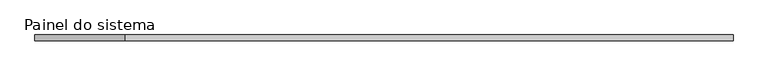
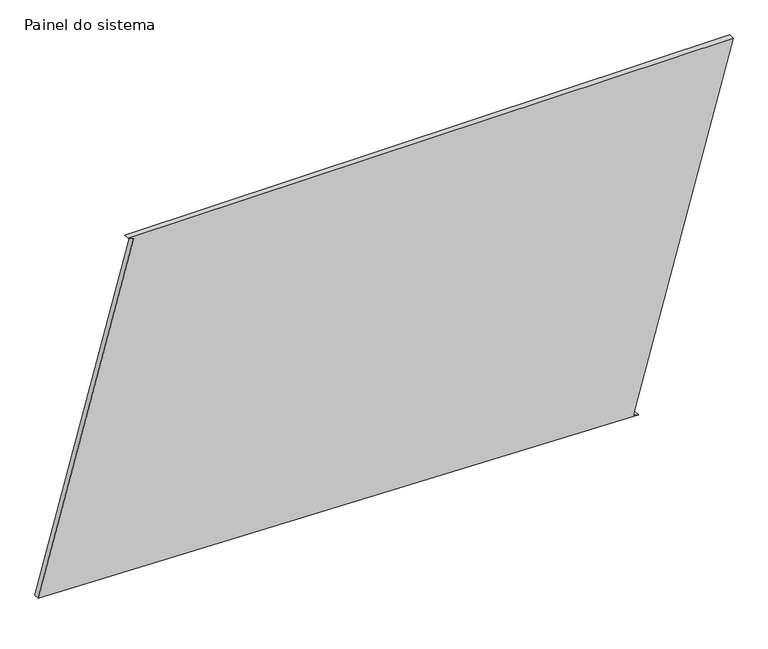
"""IFC4 building model written with IfcOpenShell, lengths in millimetres: plate geometry, Painel do sistema : Envidraçado."""

import ifcopenshell
import ifcopenshell.guid

model = None  # the IFC model being written
_history = None  # IfcOwnerHistory: only IFC2X3 demands one
_inside = {}  # id of a spatial element -> (the spatial element, [elements in it])
_under = {}  # id of a project, library or spatial element -> (it, [spatial elements below it])
_declared = {}  # id of a project -> (the project, [libraries it declares])
_typed = {}  # id of a type object -> (the type object, [elements of that type])
_made_of = {}  # id of a material, layer set ... -> (it, [elements and type objects made of it])


def new_model(schema):
    """Start an empty IFC model of exactly this schema.

    Asked for "IFC4X3", IfcOpenShell would pick the latest addendum, in which some entities
    have other attributes; the version numbers below select the first issue.
    IFC2X3 requires an IfcOwnerHistory on every rooted entity: one is made here for all.
    """
    global model, _history
    if schema == "IFC4X3":
        model = ifcopenshell.file(schema_version=(4, 3, 0, 0))
    else:
        model = ifcopenshell.file(schema=schema)
    _inside.clear()
    _under.clear()
    _declared.clear()
    _typed.clear()
    _made_of.clear()
    _history = None
    if model.schema == "IFC2X3":
        org = make("IfcOrganization", Name="unknown")
        user = make(
            "IfcPersonAndOrganization",
            ThePerson=make("IfcPerson", FamilyName="unknown"),
            TheOrganization=org,
        )
        app = make(
            "IfcApplication",
            ApplicationDeveloper=org,
            Version="unknown",
            ApplicationFullName="unknown",
            ApplicationIdentifier="unknown",
        )
        _history = make(
            "IfcOwnerHistory",
            OwningUser=user,
            OwningApplication=app,
            ChangeAction="ADDED",
            CreationDate=0,
        )
    return model


def make(cls, **values):
    """One entity of the class cls with the attributes given. An attribute that is None is left unset."""
    return model.create_entity(
        cls, **{name: value for name, value in values.items() if value is not None}
    )


def rooted(cls, **values):
    """An entity with a GlobalId (a new one), such as an element, a storey or a relation."""
    return make(cls, GlobalId=ifcopenshell.guid.new(), OwnerHistory=_history, **values)


def si_unit(unit_type, name, prefix=None):
    """IfcSIUnit, for example si_unit("LENGTHUNIT", "METRE", prefix="MILLI")."""
    return make("IfcSIUnit", UnitType=unit_type, Prefix=prefix, Name=name)


def assignment(units):
    """IfcUnitAssignment: the units of a project."""
    return None if units is None else make("IfcUnitAssignment", Units=units)


def point(xyz):
    """IfcCartesianPoint."""
    return None if xyz is None else make("IfcCartesianPoint", Coordinates=xyz)


def direction(xyz):
    """IfcDirection."""
    return None if xyz is None else make("IfcDirection", DirectionRatios=xyz)


def frame(location, z_axis=None, x_axis=None):
    """IfcAxis2Placement3D, a coordinate frame: its origin and axes. An axis left out is left unset."""
    return make(
        "IfcAxis2Placement3D",
        Location=point(location),
        Axis=direction(z_axis),
        RefDirection=direction(x_axis),
    )


def origin():
    """The frame at (0, 0, 0) with its axes left unset."""
    return frame((0.0, 0.0, 0.0))


def place(relative_to, where):
    """IfcLocalPlacement: puts the frame where relative to a parent placement (None: the world)."""
    return make(
        "IfcLocalPlacement", PlacementRelTo=relative_to, RelativePlacement=where
    )


def context(
    kind, dimensions, precision=None, world=None, true_north=None, identifier=None
):
    """IfcGeometricRepresentationContext, for example the 3D "Model" context."""
    return make(
        "IfcGeometricRepresentationContext",
        ContextIdentifier=identifier,
        ContextType=kind,
        CoordinateSpaceDimension=dimensions,
        Precision=precision,
        WorldCoordinateSystem=world,
        TrueNorth=true_north,
    )


def project(units=None, contexts=None):
    """IfcProject with its units and contexts."""
    return rooted(
        "IfcProject",
        Name="project",
        RepresentationContexts=contexts,
        UnitsInContext=assignment(units),
    )


def spatial(cls, under=None, at=None, **own):
    """A site, building, storey or space (cls), placed at a placement, below another one or the project."""
    s = rooted(cls, ObjectPlacement=at, **own)
    if under is not None:
        _under.setdefault(under.id(), (under, []))[1].append(s)
    return s


def polyline(points):
    """IfcPolyline through the points."""
    return make("IfcPolyline", Points=[point(p) for p in points])


def outline(outer, holes=None, kind="AREA"):
    """IfcArbitraryClosedProfileDef: a profile drawn as a closed curve; with holes, ...WithVoids."""
    if holes is None:
        return make("IfcArbitraryClosedProfileDef", ProfileType=kind, OuterCurve=outer)
    return make(
        "IfcArbitraryProfileDefWithVoids",
        ProfileType=kind,
        OuterCurve=outer,
        InnerCurves=holes,
    )


def extrude(swept, where, along, depth):
    """IfcExtrudedAreaSolid: the profile swept, set in the frame where, extruded along a direction by depth."""
    return make(
        "IfcExtrudedAreaSolid",
        SweptArea=swept,
        Position=where,
        ExtrudedDirection=direction(along),
        Depth=depth,
    )


def shape(context_of_items, identifier, shape_type, items):
    """IfcShapeRepresentation: the items that make up one representation, for example the "Body"."""
    return make(
        "IfcShapeRepresentation",
        ContextOfItems=context_of_items,
        RepresentationIdentifier=identifier,
        RepresentationType=shape_type,
        Items=items,
    )


def source(mapping_origin, context_of_items, identifier, shape_type, items):
    """IfcRepresentationMap: a shape defined once, which mapped items show again and again."""
    return make(
        "IfcRepresentationMap",
        MappingOrigin=mapping_origin,
        MappedRepresentation=shape(context_of_items, identifier, shape_type, items),
    )


def transform(
    local_origin,
    x_axis=None,
    y_axis=None,
    z_axis=None,
    scale=None,
    scale2=None,
    scale3=None,
    uniform=True,
):
    """IfcCartesianTransformationOperator3D, or its non-uniform kind. x_axis, y_axis, z_axis: its Axis1, 2, 3."""
    if uniform:
        return make(
            "IfcCartesianTransformationOperator3D",
            Axis1=direction(x_axis),
            Axis2=direction(y_axis),
            LocalOrigin=point(local_origin),
            Scale=scale,
            Axis3=direction(z_axis),
        )
    return make(
        "IfcCartesianTransformationOperator3DnonUniform",
        Axis1=direction(x_axis),
        Axis2=direction(y_axis),
        LocalOrigin=point(local_origin),
        Scale=scale,
        Axis3=direction(z_axis),
        Scale2=scale2,
        Scale3=scale3,
    )


def mapped(mapping_source, mapping_target):
    """IfcMappedItem: shows the shape of a source again, moved by a transform."""
    return make(
        "IfcMappedItem", MappingSource=mapping_source, MappingTarget=mapping_target
    )


def made_of(thing, what):
    """Note that an element or type object is made of a material, layer set ...; save() writes the relation."""
    if what is not None:
        _made_of.setdefault(what.id(), (what, []))[1].append(thing)
    return thing


def element(
    cls,
    number,
    at=None,
    inside=None,
    cuts=None,
    type_object=None,
    material=None,
    context=None,
    identifier="Body",
    shape_type=None,
    held_by="IfcProductDefinitionShape",
    body=None,
    shapes=None,
    **own,
):
    """One element of the class cls, such as IfcWall. Its Tag is "e" and its number.

    at: its placement. inside: the storey or other place that contains it. cuts: it is an
    opening in that element (IfcRelVoidsElement). A single representation is given by context,
    identifier, shape_type and body (its items); several are given by shapes. held_by: the class
    of the entity that holds the representations. save() writes the other relations.
    """
    e = rooted(cls, Tag="e%d" % number, ObjectPlacement=at, **own)
    if body is not None:
        shapes = [shape(context, identifier, shape_type, body)]
    if shapes is not None:
        e.Representation = make(held_by, Representations=shapes)
    if inside is not None:
        _inside.setdefault(inside.id(), (inside, []))[1].append(e)
    if cuts is not None:
        rooted(
            "IfcRelVoidsElement", RelatingBuildingElement=cuts, RelatedOpeningElement=e
        )
    if type_object is not None:
        _typed.setdefault(type_object.id(), (type_object, []))[1].append(e)
    return made_of(e, material)


def aggregate(whole, parts):
    """IfcRelAggregates: a whole, such as a stair, and the parts it consists of."""
    return rooted("IfcRelAggregates", RelatingObject=whole, RelatedObjects=parts)


def save(model, path):
    """Write the relations noted so far, then the file.

    IfcRelAggregates (storeys below a building ...), IfcRelContainedInSpatialStructure (elements
    in a storey), IfcRelDefinesByType, IfcRelAssociatesMaterial and IfcRelDeclares: one each for
    every whole, place, type object, material and project.
    """
    for whole, parts in _under.values():
        aggregate(whole, parts)
    for where, things in _inside.values():
        rooted(
            "IfcRelContainedInSpatialStructure",
            RelatedElements=things,
            RelatingStructure=where,
        )
    for kind, things in _typed.values():
        rooted("IfcRelDefinesByType", RelatedObjects=things, RelatingType=kind)
    for what, things in _made_of.values():
        rooted("IfcRelAssociatesMaterial", RelatedObjects=things, RelatingMaterial=what)
    for by, libraries in _declared.values():
        rooted("IfcRelDeclares", RelatingContext=by, RelatedDefinitions=libraries)
    model.write(path)


def painel_do_sistema_a1e68901(model_context):
    return source(origin(), model_context, "Body", "SweptSolid", [
        extrude(outline(polyline([(0.0, 1104.8531926), (6.6310485, 1080.7486454), (1595.6902398, 1517.8914202), (1595.6902398, -1124.3786442), (1589.0591912, -1100.274097), (70.9770358, -1517.8914202), (0.0, 1104.8531926)])), frame((0.0, 24.5, 0.0), z_axis=(0.0, 1.0, 0.0), x_axis=(0.0, 0.0, 1.0)), (0.0, 0.0, 1.0), 25.0),
    ])


if __name__ == "__main__":
    model = new_model("IFC4")
    model_context = context("Model", 3, world=origin())
    ifc_project = project(units=[si_unit("LENGTHUNIT", "METRE", prefix="MILLI")], contexts=[model_context])
    site = spatial("IfcSite", under=ifc_project)
    building = spatial("IfcBuilding", under=site)
    placement = place(None, origin())
    painel_do_sistema_shape = painel_do_sistema_a1e68901(model_context)
    element("IfcPlate", 1, ObjectType="Painel do sistema : Envidraçado", at=placement, inside=building, context=model_context, shape_type="MappedRepresentation", body=[
        mapped(painel_do_sistema_shape, transform((0.0, 0.0, 0.0), x_axis=(1.0, 0.0, 0.0), y_axis=(0.0, 1.0, 0.0), z_axis=(0.0, 0.0, 1.0))),
    ])
    save(model, "model.ifc")

# Revit data of these elements
# Type "Painel do sistema : Envidraçado"
#   Construction Type Id = "GSP4R"
#   Analytic Construction = "Vidraça única Pilkington 1/8 pol"
#   Visual Light Transmittance = 0.9
#   Solar Heat Gain Coefficient = 0.86
#   Heat Transfer Coefficient (U) = 6.7069 W/(m²·K)
# Element 1 (IfcPlate, "Painel do sistema : Envidraçado")
#   Materials on its faces: "Vidro"
# Materials
#   "Vidro": class "Vidro", colour RGB 0 128 192, transparency 0.9, Description = "Vidro de sílica", Cost = 0
